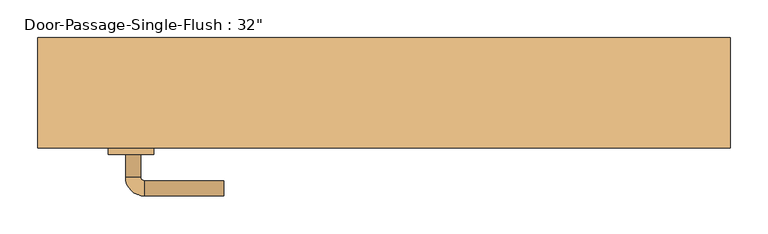
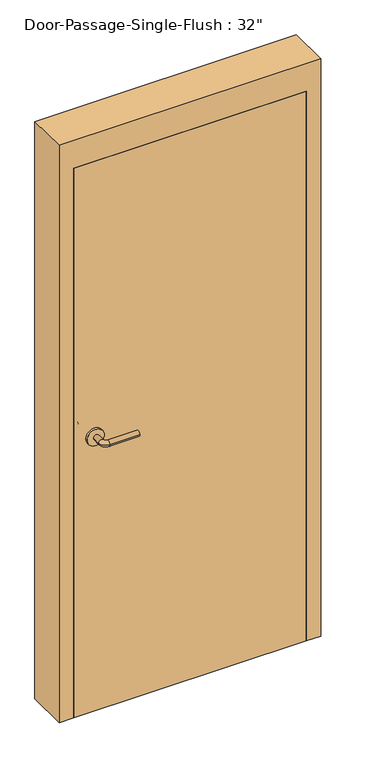
"""IFC4 building model written with IfcOpenShell, lengths in millimetres: door geometry."""

from ifc_helpers import new_model, si_unit, point, frame, frame_2d, origin, origin_with_axes, place, context, project, spatial, polyline, circle_curve, ellipse_curve, trimmed, segment, composite_curve, outline, extrude, faceted_brep, source, transform, mapped, element, save
from ifc_brep_helpers import plane_surface, cylinder_surface, revolved_surface, advanced_brep


def door_95bf5518(model_context):
    return source(origin(), model_context, "Body", "SolidModel", [
        advanced_brep(
        [(-341.390625, 11.175, 1016.0), (-321.390625, 11.175, 1016.0), (-341.390625, 41.175, 1016.0), (-321.390625, 41.175, 1016.0), (-316.390625, 46.175, 1016.0), (-316.390625, 66.175, 1016.0), (-211.390625, 66.175, 1016.0), (-211.390625, 46.175, 1016.0)],
        [
            (0, 1, circle_curve(frame((-331.390625, 11.175, 1016.0), z_axis=(0.0, -1.0, 0.0), x_axis=(1.0, 0.0, 0.0)), 10.0)),
            (1, 0, circle_curve(frame((-331.390625, 11.175, 1016.0), z_axis=(0.0, -1.0, 0.0), x_axis=(1.0, 0.0, 0.0)), 10.0)),
            (0, 2),
            (2, 3, circle_curve(frame((-331.390625, 41.175, 1016.0), z_axis=(0.0, -1.0, 0.0), x_axis=(1.0, 0.0, 0.0)), 10.0)),
            (3, 1),
            (3, 2, circle_curve(frame((-331.390625, 41.175, 1016.0), z_axis=(0.0, -1.0, 0.0), x_axis=(1.0, 0.0, 0.0)), 10.0)),
            (4, 3, circle_curve(frame((-316.390625, 41.175, 1016.0), z_axis=(0.0, 0.0, 1.0), x_axis=(-1.0, 0.0, 0.0)), 5.0)),
            (2, 5, circle_curve(frame((-316.390625, 41.175, 1016.0), z_axis=(0.0, 0.0, -1.0), x_axis=(-1.0, 0.0, 0.0)), 25.0)),
            (5, 4, circle_curve(frame((-316.390625, 56.175, 1016.0), z_axis=(-1.0, 0.0, 0.0), x_axis=(0.0, -1.0, 0.0)), 10.0)),
            (4, 5, circle_curve(frame((-316.390625, 56.175, 1016.0), z_axis=(-1.0, 0.0, 0.0), x_axis=(0.0, -1.0, 0.0)), 10.0)),
            (6, 7, circle_curve(frame((-211.390625, 56.175, 1016.0), z_axis=(1.0, 0.0, 0.0), x_axis=(0.0, -1.0, 0.0)), 10.0)),
            (7, 6, circle_curve(frame((-211.390625, 56.175, 1016.0), z_axis=(1.0, 0.0, 0.0), x_axis=(0.0, -1.0, 0.0)), 10.0)),
            (5, 6),
            (7, 4),
        ],
        [
            plane_surface(frame((-331.390625, 11.175, 1016.0), z_axis=(0.0, -1.0, 0.0), x_axis=(0.0, 0.0, 1.0))),
            cylinder_surface(frame((-331.390625, 11.175, 1016.0), z_axis=(0.0, -1.0, 0.0), x_axis=(1.0, 0.0, 0.0)), 10.0),
            revolved_surface(trimmed(ellipse_curve(frame((-331.390625, 41.175, 1016.0), z_axis=(0.0, -1.0, 0.0), x_axis=(1.0, 0.0, 0.0)), 10.0, 10.0), [point((-341.390625, 41.175, 1016.0))], [point((-321.390625, 41.175, 1016.0))], True, "CARTESIAN"), (-316.390625, 41.175, 1016.0), (0.0, 0.0, -1.0)),
            revolved_surface(trimmed(ellipse_curve(frame((-331.390625, 41.175, 1016.0), z_axis=(0.0, -1.0, 0.0), x_axis=(1.0, 0.0, 0.0)), 10.0, 10.0), [point((-321.390625, 41.175, 1016.0))], [point((-341.390625, 41.175, 1016.0))], True, "CARTESIAN"), (-316.390625, 41.175, 1016.0), (0.0, 0.0, -1.0)),
            plane_surface(frame((-211.390625, 56.175, 1016.0), z_axis=(1.0, 0.0, 0.0), x_axis=(0.0, 0.0, 1.0))),
            cylinder_surface(frame((-316.390625, 56.175, 1016.0), z_axis=(-1.0, 0.0, 0.0), x_axis=(0.0, -1.0, 0.0)), 10.0),
        ],
        [
            (0, [[1, 2]]),
            (1, [[-1, 3, 4, 5]]),
            (1, [[-2, -5, 6, -3]]),
            (2, [[7, -4, 8, 9]]),
            (3, [[-8, -6, -7, 10]]),
            (4, [[11, 12]]),
            (5, [[-9, 13, -12, 14]]),
            (5, [[-10, -14, -11, -13]]),
        ],
    ),
        extrude(outline(composite_curve([segment(trimmed(circle_curve(frame_2d((1016.0, -333.890625)), 30.0), [point((1016.0, -363.890625))], [point((1016.0, -303.890625))], False, "CARTESIAN"), True, "CONTINUOUS"), segment(trimmed(circle_curve(frame_2d((1016.0, -333.890625)), 30.0), [point((1016.0, -303.890625))], [point((1016.0, -363.890625))], False, "CARTESIAN"), True, "CONTINUOUS")], self_intersect=False)), frame((0.0, 3.175, 0.0), z_axis=(0.0, 1.0, 0.0), x_axis=(0.0, 0.0, 1.0)), (0.0, 0.0, 1.0), 8.0),
        advanced_brep(
        [(-341.390625, -49.275, 1016.0), (-321.390625, -49.275, 1016.0), (-321.390625, -79.275, 1016.0), (-341.390625, -79.275, 1016.0), (-316.390625, -84.275, 1016.0), (-316.390625, -104.275, 1016.0), (-211.390625, -104.275, 1016.0), (-211.390625, -84.275, 1016.0)],
        [
            (0, 1, circle_curve(frame((-331.390625, -49.275, 1016.0), z_axis=(0.0, 1.0, 0.0), x_axis=(1.0, 0.0, 0.0)), 10.0)),
            (1, 0, circle_curve(frame((-331.390625, -49.275, 1016.0), z_axis=(0.0, 1.0, 0.0), x_axis=(1.0, 0.0, 0.0)), 10.0)),
            (1, 2),
            (2, 3, circle_curve(frame((-331.390625, -79.275, 1016.0), z_axis=(0.0, 1.0, 0.0), x_axis=(1.0, 0.0, 0.0)), 10.0)),
            (3, 0),
            (3, 2, circle_curve(frame((-331.390625, -79.275, 1016.0), z_axis=(0.0, 1.0, 0.0), x_axis=(1.0, 0.0, 0.0)), 10.0)),
            (4, 5, circle_curve(frame((-316.390625, -94.275, 1016.0), z_axis=(-1.0, 0.0, 0.0), x_axis=(0.0, 1.0, 0.0)), 10.0)),
            (5, 3, circle_curve(frame((-316.390625, -79.275, 1016.0), z_axis=(0.0, 0.0, -1.0), x_axis=(-1.0, 0.0, 0.0)), 25.0)),
            (2, 4, circle_curve(frame((-316.390625, -79.275, 1016.0), z_axis=(0.0, 0.0, 1.0), x_axis=(-1.0, 0.0, 0.0)), 5.0)),
            (5, 4, circle_curve(frame((-316.390625, -94.275, 1016.0), z_axis=(-1.0, 0.0, 0.0), x_axis=(0.0, 1.0, 0.0)), 10.0)),
            (6, 7, circle_curve(frame((-211.390625, -94.275, 1016.0), z_axis=(1.0, 0.0, 0.0), x_axis=(0.0, 1.0, 0.0)), 10.0)),
            (7, 6, circle_curve(frame((-211.390625, -94.275, 1016.0), z_axis=(1.0, 0.0, 0.0), x_axis=(0.0, 1.0, 0.0)), 10.0)),
            (4, 7),
            (6, 5),
        ],
        [
            plane_surface(frame((-331.390625, -49.275, 1016.0), z_axis=(0.0, 1.0, 0.0), x_axis=(0.0, 0.0, 1.0))),
            cylinder_surface(frame((-331.390625, -49.275, 1016.0), z_axis=(0.0, 1.0, 0.0), x_axis=(1.0, 0.0, 0.0)), 10.0),
            revolved_surface(trimmed(ellipse_curve(frame((-331.390625, -79.275, 1016.0), z_axis=(0.0, -1.0, 0.0), x_axis=(1.0, 0.0, 0.0)), 10.0, 10.0), [point((-341.390625, -79.275, 1016.0))], [point((-321.390625, -79.275, 1016.0))], True, "CARTESIAN"), (-316.390625, -79.275, 1016.0), (0.0, 0.0, -1.0)),
            revolved_surface(trimmed(ellipse_curve(frame((-331.390625, -79.275, 1016.0), z_axis=(0.0, -1.0, 0.0), x_axis=(1.0, 0.0, 0.0)), 10.0, 10.0), [point((-321.390625, -79.275, 1016.0))], [point((-341.390625, -79.275, 1016.0))], True, "CARTESIAN"), (-316.390625, -79.275, 1016.0), (0.0, 0.0, -1.0)),
            plane_surface(frame((-211.390625, -94.275, 1016.0), z_axis=(1.0, 0.0, 0.0), x_axis=(0.0, 0.0, 1.0))),
            cylinder_surface(frame((-316.390625, -94.275, 1016.0), z_axis=(-1.0, 0.0, 0.0), x_axis=(0.0, 1.0, 0.0)), 10.0),
        ],
        [
            (0, [[1, 2]]),
            (1, [[3, 4, 5, -2]]),
            (1, [[-5, 6, -3, -1]]),
            (2, [[7, 8, -4, 9]]),
            (3, [[10, -9, -6, -8]]),
            (4, [[11, 12]]),
            (5, [[13, -11, 14, -7]]),
            (5, [[-14, -12, -13, -10]]),
        ],
    ),
        extrude(outline(composite_curve([segment(trimmed(circle_curve(frame_2d((1016.0, -333.890625)), 30.0), [point((1016.0, -363.890625))], [point((1016.0, -303.890625))], False, "CARTESIAN"), True, "CONTINUOUS"), segment(trimmed(circle_curve(frame_2d((1016.0, -333.890625)), 30.0), [point((1016.0, -303.890625))], [point((1016.0, -363.890625))], False, "CARTESIAN"), True, "CONTINUOUS")], self_intersect=False)), frame((0.0, -49.275, 0.0), z_axis=(0.0, 1.0, 0.0), x_axis=(0.0, 0.0, 1.0)), (0.0, 0.0, 1.0), 8.0),
        faceted_brep([(406.4, 7.9375, 0.0), (390.525, 7.9375, 0.0), (390.525, 55.5625, 0.0), (406.4, 55.5625, 0.0), (406.4, 104.775, 0.0), (457.2, 104.775, 0.0), (457.2, -41.275, 0.0), (406.4, -41.275, 0.0), (406.4, -41.275, 2032.0), (406.4, 7.9375, 2032.0), (457.2, -41.275, 2133.6), (-457.2, -41.275, 2133.6), (-457.2, -41.275, 0.0), (-406.4, -41.275, 0.0), (-406.4, -41.275, 2032.0), (457.2, 104.775, 2133.6), (406.4, 104.775, 2032.0), (-406.4, 104.775, 2032.0), (-406.4, 104.775, 0.0), (-457.2, 104.775, 0.0), (-457.2, 104.775, 2133.6), (406.4, 55.5625, 2032.0), (390.525, 55.5625, 2016.125), (-390.525, 55.5625, 2016.125), (-390.525, 55.5625, 0.0), (-406.4, 55.5625, 0.0), (-406.4, 55.5625, 2032.0), (390.525, 7.9375, 2016.125), (-406.4, 7.9375, 2032.0), (-406.4, 7.9375, 0.0), (-390.525, 7.9375, 0.0), (-390.525, 7.9375, 2016.125)], [[[0, 1, 2, 3, 4, 5, 6, 7]], [[7, 8, 9, 0]], [[6, 10, 11, 12, 13, 14, 8, 7]], [[5, 15, 10, 6]], [[4, 16, 17, 18, 19, 20, 15, 5]], [[3, 21, 16, 4]], [[2, 22, 23, 24, 25, 26, 21, 3]], [[1, 27, 22, 2]], [[0, 9, 28, 29, 30, 31, 27, 1]], [[8, 14, 28, 9]], [[16, 21, 26, 17]], [[22, 27, 31, 23]], [[12, 19, 18, 25, 24, 30, 29, 13]], [[13, 29, 28, 14]], [[11, 20, 19, 12]], [[17, 26, 25, 18]], [[23, 31, 30, 24]], [[15, 20, 11, 10]]]),
        extrude(outline(polyline([(406.4, 3.175), (406.4, -41.275), (-406.4, -41.275), (-406.4, 3.175), (406.4, 3.175)])), origin_with_axes(), (0.0, 0.0, 1.0), 2032.0),
    ])


if __name__ == "__main__":
    model = new_model("IFC4")
    model_context = context("Model", 3, world=origin())
    ifc_project = project(units=[si_unit("LENGTHUNIT", "METRE", prefix="MILLI")], contexts=[model_context])
    site = spatial("IfcSite", under=ifc_project)
    building = spatial("IfcBuilding", under=site)
    placement = place(None, origin())
    door_shape = door_95bf5518(model_context)
    element("IfcDoor", 1, ObjectType="Door-Passage-Single-Flush : 32\"", at=placement, inside=building, context=model_context, shape_type="MappedRepresentation", body=[
        mapped(door_shape, transform((0.0, 0.0, 0.0), x_axis=(1.0, 0.0, 0.0), y_axis=(0.0, 1.0, 0.0), z_axis=(0.0, 0.0, 1.0))),
    ])
    save(model, "model.ifc")

# Revit data of these elements
# Type "Door-Passage-Single-Flush : 32\""
#   Type Mark = "42"
#   Assembly Code = "B2030200"
#   Analytic Construction = "Wooden"
#   Thickness = 0' - 1 3/4"
#   Thermal Resistance (R) = 0.455703 (m²·K)/W
#   Swing Angle [instance default] = 90.00°
#   Strike Height = 3' - 4"
#   Rough Width [instance default] = 3' - 0"
#   Rough Height [instance default] = 7' - 0"
#   MF Opening Height [instance default] = 0' - 4"
#   MF Opening Width [instance default] = 0' - 4"
#   Inset Calculate [instance default] = 0' - 4"
#   Masonry Inset [instance default] = 0' - 1"
#   Height = 6' - 8"
#   Width = 2' - 8"
#   Heat Transfer Coefficient (U) = 2.19465 W/(m²·K)
#   Masonry Frame Depth = 0' - 5 3/4"
#   Masonry Frame [instance default] = yes
#   Function = 1
#   Dry Wall Frame [instance default] = no
#   Panel Material = Wood - Birch
#   Frame Material = Metal - Paint Finish - Grey
#   Door Handle Material = Aluminum
#   Visual Light Transmittance = 0
#   Solar Heat Gain Coefficient = 0
#   Wall Closure = (empty or 0)
# Element 1 (IfcDoor, "Door-Passage-Single-Flush : 32\"")
#   Materials on its faces: "Aluminum", "Metal - Paint Finish - Grey", "Wood - Birch"
# Materials
#   "Wood - Birch": class "Wood", colour RGB 166 116 52, transparency 0, Cost = 0
#   "Metal - Paint Finish - Grey": class "Paint", colour RGB 104 104 104, transparency 0, Cost = 0
#   "Aluminum": class "Metal", colour RGB 247 247 247, transparency 0, Description = "Aluminum 6061", Cost = 0
